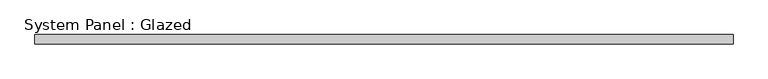
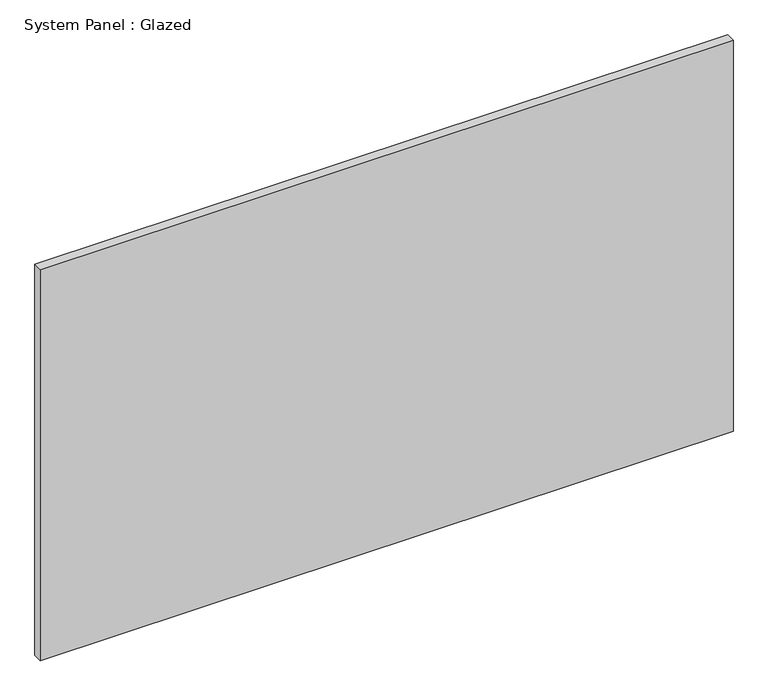
"""IFC4 building model written with IfcOpenShell, lengths in millimetres: plate geometry, System Panel : Glazed."""

from ifc_helpers import new_model, si_unit, origin, origin_with_axes, place, context, project, spatial, polyline, outline, extrude, source, transform, mapped, element, save


def system_panel_glazed_576e2b42(model_context):
    return source(origin(), model_context, "Body", "SweptSolid", [
        extrude(outline(polyline([(968.375, 19.05), (-968.375, 19.05), (-968.375, 44.45), (968.375, 44.45), (968.375, 19.05)])), origin_with_axes(), (0.0, 0.0, 1.0), 1155.7),
    ])


if __name__ == "__main__":
    model = new_model("IFC4")
    model_context = context("Model", 3, world=origin())
    ifc_project = project(units=[si_unit("LENGTHUNIT", "METRE", prefix="MILLI")], contexts=[model_context])
    site = spatial("IfcSite", under=ifc_project)
    building = spatial("IfcBuilding", under=site)
    placement = place(None, origin())
    system_panel_glazed_shape = system_panel_glazed_576e2b42(model_context)
    element("IfcPlate", 1, ObjectType="System Panel : Glazed", at=placement, inside=building, context=model_context, shape_type="MappedRepresentation", body=[
        mapped(system_panel_glazed_shape, transform((0.0, 0.0, 0.0), x_axis=(1.0, 0.0, 0.0), y_axis=(0.0, 1.0, 0.0), z_axis=(0.0, 0.0, 1.0))),
    ])
    save(model, "model.ifc")

# Revit data of these elements
# Element 1 (IfcPlate, "System Panel : Glazed")
#   Materials on its faces: "Glass"
# Materials
#   "Glass": class "Glass", colour RGB 0 128 192, transparency 0.75
